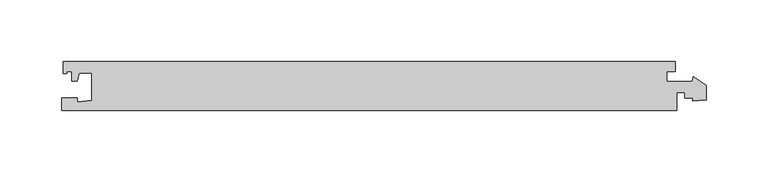
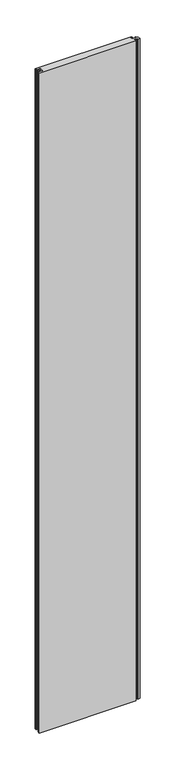
"""IFC4 building model written with IfcOpenShell, lengths in millimetres: proxy geometry, Generic Models 5:Generic Models 5:321804:Generic Models 5:321804 : Generic Models 5:Generic Models 5:321804:31 : Generic Models 5:Generic Models 5:321804:Generic Models 5:321804 : Generic Models 5:Generic Models 5:321804:300761."""

from ifc_helpers import new_model, si_unit, frame, origin, place, context, project, spatial, polyline, outline, extrude, source, transform, mapped, element, save


def generic_models_a86e09e5(model_context):
    return source(origin(), model_context, "Body", "SweptSolid", [
        extrude(outline(polyline([(594965.7852942, -579052.1037319), (594964.0436245, -579058.6037319), (594959.5936245, -579058.6037319), (594959.5936245, -579051.1037319), (594955.6436245, -579051.1037319), (594955.6436245, -579052.6037319), (594952.6436245, -579052.6037319), (594952.6436245, -579042.6037319), (595450.1436245, -579042.6037319), (595450.1436245, -579051.1037319), (595443.1936245, -579051.1037319), (595443.1936245, -579059.1037319), (595463.9096499, -579059.1037319), (595464.9621226, -579055.1758504), (595475.6436245, -579062.2832156), (595475.6436245, -579074.1413566), (595464.6436245, -579075.1037319), (595464.6436245, -579072.4037319), (595458.0186245, -579072.4037319), (595458.0186245, -579068.1037319), (595451.3936245, -579068.1037319), (595451.3936245, -579082.6037319), (594951.3936245, -579082.6037319), (594951.3936245, -579072.4037319), (594964.1436245, -579072.4037319), (594964.1436245, -579075.6493861), (594976.1436245, -579074.5995222), (594976.1436245, -579052.1037319), (594965.7852942, -579052.1037319)])), frame((0.0, 0.0, 54.8767776), z_axis=(0.0, 0.0, 1.0), x_axis=(1.0, 0.0, 0.0)), (0.0, 0.0, 1.0), 3595.9825169),
    ])


if __name__ == "__main__":
    model = new_model("IFC4")
    model_context = context("Model", 3, world=origin())
    ifc_project = project(units=[si_unit("LENGTHUNIT", "METRE", prefix="MILLI")], contexts=[model_context])
    site = spatial("IfcSite", under=ifc_project)
    building = spatial("IfcBuilding", under=site)
    placement = place(None, origin())
    generic_models_shape = generic_models_a86e09e5(model_context)
    element("IfcBuildingElementProxy", 1, Name="Generic Models 5:Generic Models 5:321804:Generic Models 5:321804 : Generic Models 5:Generic Models 5:321804:31 : Generic Models 5:Generic Models 5:321804:Generic Models 5:321804 : Generic Models 5:Generic Models 5:321804:300761", ObjectType="Generic Models 5:Generic Models 5:321804:Generic Models 5:321804 : Generic Models 5:Generic Models 5:321804:31 : Generic Models 5:Generic Models 5:321804:Generic Models 5:321804 : Generic Models 5:Generic Models 5:321804:300761", at=placement, inside=building, context=model_context, shape_type="MappedRepresentation", body=[
        mapped(generic_models_shape, transform((0.0, 0.0, 0.0), x_axis=(1.0, 0.0, 0.0), y_axis=(0.0, 1.0, 0.0), z_axis=(0.0, 0.0, 1.0))),
    ])
    save(model, "model.ifc")

# Revit data of these elements
# Type "Generic Models 5:Generic Models 5:321804:Generic Models 5:321804 : Generic Models 5:Generic Models 5:321804:31 : Generic Models 5:Generic Models 5:321804:Generic Models 5:321804 : Generic Models 5:Generic Models 5:321804:300761"
#   NameOverride = "Generic Models 5:Generic Models 5:321804:Generic Models 5:321804 : Generic Models 5:Generic Models 5:321804:300761"
#   ObjectTypeOverride = "Generic Models 5:321804 : Generic Models 5:Generic Models 5:321804"
#   Reference = "Generic Models 5"
#   Tag = "300761"
# Element 1 (IfcBuildingElementProxy, "Generic Models 5:Generic Models 5:321804:Generic Models 5:321804 : Generic Models 5:Generic Models 5:321804:31 : Generic Models 5:Generic Models 5:321804:Generic Models 5:321804 : Generic Models 5:Generic Models 5:321804:300761")
#   Materials on its faces: "POLYCARBONATE PANEL - ARCOPLUS 547"
# Materials
#   "POLYCARBONATE PANEL - ARCOPLUS 547": class "Unassigned", colour RGB 202 225 249, transparency 0.45, Cost = 0
